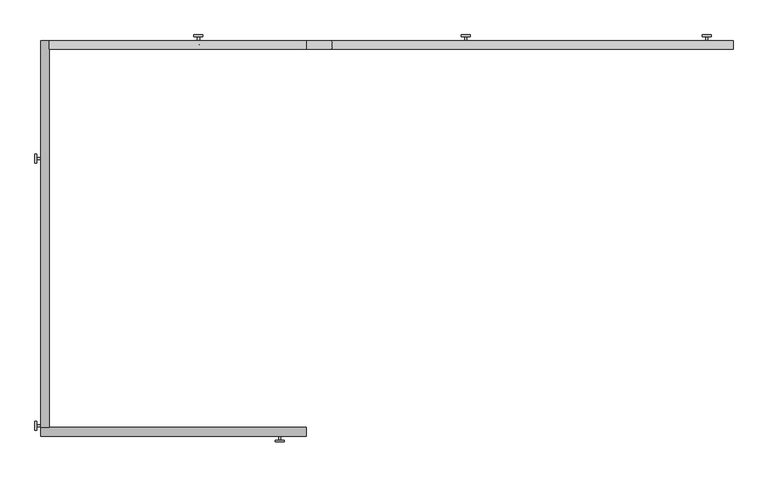
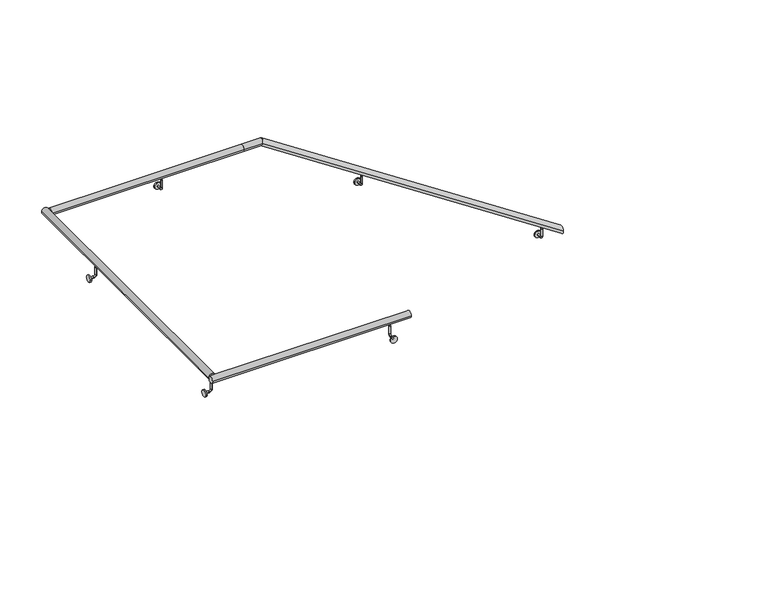
"""IFC4 building model written with IfcOpenShell, lengths in millimetres: railing geometry."""

import ifcopenshell
import ifcopenshell.guid

model = None  # the IFC model being written
_history = None  # IfcOwnerHistory: only IFC2X3 demands one
_inside = {}  # id of a spatial element -> (the spatial element, [elements in it])
_under = {}  # id of a project, library or spatial element -> (it, [spatial elements below it])
_declared = {}  # id of a project -> (the project, [libraries it declares])
_typed = {}  # id of a type object -> (the type object, [elements of that type])
_made_of = {}  # id of a material, layer set ... -> (it, [elements and type objects made of it])


def new_model(schema):
    """Start an empty IFC model of exactly this schema.

    Asked for "IFC4X3", IfcOpenShell would pick the latest addendum, in which some entities
    have other attributes; the version numbers below select the first issue.
    IFC2X3 requires an IfcOwnerHistory on every rooted entity: one is made here for all.
    """
    global model, _history
    if schema == "IFC4X3":
        model = ifcopenshell.file(schema_version=(4, 3, 0, 0))
    else:
        model = ifcopenshell.file(schema=schema)
    _inside.clear()
    _under.clear()
    _declared.clear()
    _typed.clear()
    _made_of.clear()
    _history = None
    if model.schema == "IFC2X3":
        org = make("IfcOrganization", Name="unknown")
        user = make(
            "IfcPersonAndOrganization",
            ThePerson=make("IfcPerson", FamilyName="unknown"),
            TheOrganization=org,
        )
        app = make(
            "IfcApplication",
            ApplicationDeveloper=org,
            Version="unknown",
            ApplicationFullName="unknown",
            ApplicationIdentifier="unknown",
        )
        _history = make(
            "IfcOwnerHistory",
            OwningUser=user,
            OwningApplication=app,
            ChangeAction="ADDED",
            CreationDate=0,
        )
    return model


def make(cls, **values):
    """One entity of the class cls with the attributes given. An attribute that is None is left unset."""
    return model.create_entity(
        cls, **{name: value for name, value in values.items() if value is not None}
    )


def rooted(cls, **values):
    """An entity with a GlobalId (a new one), such as an element, a storey or a relation."""
    return make(cls, GlobalId=ifcopenshell.guid.new(), OwnerHistory=_history, **values)


def si_unit(unit_type, name, prefix=None):
    """IfcSIUnit, for example si_unit("LENGTHUNIT", "METRE", prefix="MILLI")."""
    return make("IfcSIUnit", UnitType=unit_type, Prefix=prefix, Name=name)


def assignment(units):
    """IfcUnitAssignment: the units of a project."""
    return None if units is None else make("IfcUnitAssignment", Units=units)


def point(xyz):
    """IfcCartesianPoint."""
    return None if xyz is None else make("IfcCartesianPoint", Coordinates=xyz)


def direction(xyz):
    """IfcDirection."""
    return None if xyz is None else make("IfcDirection", DirectionRatios=xyz)


def frame(location, z_axis=None, x_axis=None):
    """IfcAxis2Placement3D, a coordinate frame: its origin and axes. An axis left out is left unset."""
    return make(
        "IfcAxis2Placement3D",
        Location=point(location),
        Axis=direction(z_axis),
        RefDirection=direction(x_axis),
    )


def frame_2d(location, x_axis=None):
    """IfcAxis2Placement2D, a coordinate frame in the plane: its origin and x axis."""
    return make(
        "IfcAxis2Placement2D", Location=point(location), RefDirection=direction(x_axis)
    )


def origin():
    """The frame at (0, 0, 0) with its axes left unset."""
    return frame((0.0, 0.0, 0.0))


def place(relative_to, where):
    """IfcLocalPlacement: puts the frame where relative to a parent placement (None: the world)."""
    return make(
        "IfcLocalPlacement", PlacementRelTo=relative_to, RelativePlacement=where
    )


def context(
    kind, dimensions, precision=None, world=None, true_north=None, identifier=None
):
    """IfcGeometricRepresentationContext, for example the 3D "Model" context."""
    return make(
        "IfcGeometricRepresentationContext",
        ContextIdentifier=identifier,
        ContextType=kind,
        CoordinateSpaceDimension=dimensions,
        Precision=precision,
        WorldCoordinateSystem=world,
        TrueNorth=true_north,
    )


def project(units=None, contexts=None):
    """IfcProject with its units and contexts."""
    return rooted(
        "IfcProject",
        Name="project",
        RepresentationContexts=contexts,
        UnitsInContext=assignment(units),
    )


def spatial(cls, under=None, at=None, **own):
    """A site, building, storey or space (cls), placed at a placement, below another one or the project."""
    s = rooted(cls, ObjectPlacement=at, **own)
    if under is not None:
        _under.setdefault(under.id(), (under, []))[1].append(s)
    return s


def circle_curve(where, radius):
    """IfcCircle in the frame where."""
    return make("IfcCircle", Position=where, Radius=radius)


def ellipse_curve(where, semi_axis1, semi_axis2):
    """IfcEllipse in the frame where."""
    return make(
        "IfcEllipse", Position=where, SemiAxis1=semi_axis1, SemiAxis2=semi_axis2
    )


def trimmed(basis, trim1, trim2, sense, master):
    """IfcTrimmedCurve: the piece of a basis curve between two trims."""
    return make(
        "IfcTrimmedCurve",
        BasisCurve=basis,
        Trim1=trim1,
        Trim2=trim2,
        SenseAgreement=sense,
        MasterRepresentation=master,
    )


def segment(curve, same_sense, transition):
    """IfcCompositeCurveSegment."""
    return make(
        "IfcCompositeCurveSegment",
        Transition=transition,
        SameSense=same_sense,
        ParentCurve=curve,
    )


def composite_curve(segments, self_intersect=None):
    """IfcCompositeCurve: segments joined end to end."""
    return make("IfcCompositeCurve", Segments=segments, SelfIntersect=self_intersect)


def outline(outer, holes=None, kind="AREA"):
    """IfcArbitraryClosedProfileDef: a profile drawn as a closed curve; with holes, ...WithVoids."""
    if holes is None:
        return make("IfcArbitraryClosedProfileDef", ProfileType=kind, OuterCurve=outer)
    return make(
        "IfcArbitraryProfileDefWithVoids",
        ProfileType=kind,
        OuterCurve=outer,
        InnerCurves=holes,
    )


def extrude(swept, where, along, depth):
    """IfcExtrudedAreaSolid: the profile swept, set in the frame where, extruded along a direction by depth."""
    return make(
        "IfcExtrudedAreaSolid",
        SweptArea=swept,
        Position=where,
        ExtrudedDirection=direction(along),
        Depth=depth,
    )


def shape(context_of_items, identifier, shape_type, items):
    """IfcShapeRepresentation: the items that make up one representation, for example the "Body"."""
    return make(
        "IfcShapeRepresentation",
        ContextOfItems=context_of_items,
        RepresentationIdentifier=identifier,
        RepresentationType=shape_type,
        Items=items,
    )


def source(mapping_origin, context_of_items, identifier, shape_type, items):
    """IfcRepresentationMap: a shape defined once, which mapped items show again and again."""
    return make(
        "IfcRepresentationMap",
        MappingOrigin=mapping_origin,
        MappedRepresentation=shape(context_of_items, identifier, shape_type, items),
    )


def transform(
    local_origin,
    x_axis=None,
    y_axis=None,
    z_axis=None,
    scale=None,
    scale2=None,
    scale3=None,
    uniform=True,
):
    """IfcCartesianTransformationOperator3D, or its non-uniform kind. x_axis, y_axis, z_axis: its Axis1, 2, 3."""
    if uniform:
        return make(
            "IfcCartesianTransformationOperator3D",
            Axis1=direction(x_axis),
            Axis2=direction(y_axis),
            LocalOrigin=point(local_origin),
            Scale=scale,
            Axis3=direction(z_axis),
        )
    return make(
        "IfcCartesianTransformationOperator3DnonUniform",
        Axis1=direction(x_axis),
        Axis2=direction(y_axis),
        LocalOrigin=point(local_origin),
        Scale=scale,
        Axis3=direction(z_axis),
        Scale2=scale2,
        Scale3=scale3,
    )


def mapped(mapping_source, mapping_target):
    """IfcMappedItem: shows the shape of a source again, moved by a transform."""
    return make(
        "IfcMappedItem", MappingSource=mapping_source, MappingTarget=mapping_target
    )


def made_of(thing, what):
    """Note that an element or type object is made of a material, layer set ...; save() writes the relation."""
    if what is not None:
        _made_of.setdefault(what.id(), (what, []))[1].append(thing)
    return thing


def element(
    cls,
    number,
    at=None,
    inside=None,
    cuts=None,
    type_object=None,
    material=None,
    context=None,
    identifier="Body",
    shape_type=None,
    held_by="IfcProductDefinitionShape",
    body=None,
    shapes=None,
    **own,
):
    """One element of the class cls, such as IfcWall. Its Tag is "e" and its number.

    at: its placement. inside: the storey or other place that contains it. cuts: it is an
    opening in that element (IfcRelVoidsElement). A single representation is given by context,
    identifier, shape_type and body (its items); several are given by shapes. held_by: the class
    of the entity that holds the representations. save() writes the other relations.
    """
    e = rooted(cls, Tag="e%d" % number, ObjectPlacement=at, **own)
    if body is not None:
        shapes = [shape(context, identifier, shape_type, body)]
    if shapes is not None:
        e.Representation = make(held_by, Representations=shapes)
    if inside is not None:
        _inside.setdefault(inside.id(), (inside, []))[1].append(e)
    if cuts is not None:
        rooted(
            "IfcRelVoidsElement", RelatingBuildingElement=cuts, RelatedOpeningElement=e
        )
    if type_object is not None:
        _typed.setdefault(type_object.id(), (type_object, []))[1].append(e)
    return made_of(e, material)


def aggregate(whole, parts):
    """IfcRelAggregates: a whole, such as a stair, and the parts it consists of."""
    return rooted("IfcRelAggregates", RelatingObject=whole, RelatedObjects=parts)


def save(model, path):
    """Write the relations noted so far, then the file.

    IfcRelAggregates (storeys below a building ...), IfcRelContainedInSpatialStructure (elements
    in a storey), IfcRelDefinesByType, IfcRelAssociatesMaterial and IfcRelDeclares: one each for
    every whole, place, type object, material and project.
    """
    for whole, parts in _under.values():
        aggregate(whole, parts)
    for where, things in _inside.values():
        rooted(
            "IfcRelContainedInSpatialStructure",
            RelatedElements=things,
            RelatingStructure=where,
        )
    for kind, things in _typed.values():
        rooted("IfcRelDefinesByType", RelatedObjects=things, RelatingType=kind)
    for what, things in _made_of.values():
        rooted("IfcRelAssociatesMaterial", RelatedObjects=things, RelatingMaterial=what)
    for by, libraries in _declared.values():
        rooted("IfcRelDeclares", RelatingContext=by, RelatedDefinitions=libraries)
    model.write(path)


def plane_surface(at):
    """IfcPlane: the flat surface through the origin of the frame at, square to its z axis."""
    return make("IfcPlane", Position=at)


def cylinder_surface(at, radius):
    """IfcCylindricalSurface: all points at the distance radius from the z axis of the frame at."""
    return make("IfcCylindricalSurface", Position=at, Radius=radius)


def revolved_surface(curve, axis_point, axis_direction):
    """IfcSurfaceOfRevolution: the curve turned about the line through axis_point along axis_direction."""
    return make(
        "IfcSurfaceOfRevolution",
        SweptCurve=make("IfcArbitraryOpenProfileDef", ProfileType="CURVE", Curve=curve),
        AxisPosition=make("IfcAxis1Placement", Location=point(axis_point), Axis=direction(axis_direction)),
    )


def advanced_brep(points, edges, surfaces, faces):
    """IfcAdvancedBrep: a solid bounded by faces that lie on surfaces and meet in shared edges.

    An edge is (start, end): straight between two places in points (the first is 0);
    or (start, end, curve); or (start, end, curve, False) where it runs against its curve.
    A face is (place in surfaces, loops), or (place, loops, False) where it looks against
    its surface's normal. A loop lists edges by number (the first is 1), with a minus sign
    where the edge is run from its end to its start. The first loop is the outer one.
    """
    corners = [point(p) for p in points]
    vertices = [make("IfcVertexPoint", VertexGeometry=c) for c in corners]
    made = []
    for start, end, *more in edges:
        made.append(
            make(
                "IfcEdgeCurve",
                EdgeStart=vertices[start],
                EdgeEnd=vertices[end],
                EdgeGeometry=more[0] if more else make("IfcPolyline", Points=[corners[start], corners[end]]),
                SameSense=more[1] if len(more) > 1 else True,
            )
        )
    hull = []
    for where, loops, *sense in faces:
        bounds = []
        for j, loop in enumerate(loops):
            ring = [make("IfcOrientedEdge", EdgeElement=made[abs(k) - 1], Orientation=k > 0) for k in loop]
            bounds.append(
                make(
                    "IfcFaceOuterBound" if j == 0 else "IfcFaceBound",
                    Bound=make("IfcEdgeLoop", EdgeList=ring),
                    Orientation=True,
                )
            )
        hull.append(make("IfcAdvancedFace", Bounds=bounds, FaceSurface=surfaces[where], SameSense=sense[0] if sense else True))
    return make("IfcAdvancedBrep", Outer=make("IfcClosedShell", CfsFaces=hull))


def railing_9a7f1ff8(model_context):
    return source(origin(), model_context, "Body", "SolidModel", [
        advanced_brep(
        [(-47571.8499394, -5172.6994487, 1246.5391039), (-47571.8499394, -5122.6994487, 1246.5391039), (-49859.4499252, -5172.6994487, 2752.7777778), (-49859.4499252, -5122.6994487, 2752.7777778), (-50001.8499394, -5172.6994487, 2752.7777778), (-50001.8499394, -5122.6994487, 2752.7777778)],
        [
            (0, 1, ellipse_curve(frame((-47571.8499394, -5147.6994487, 1246.5391039), z_axis=(1.0, 0.0, 0.0), x_axis=(0.0, 0.0, -1.0)), 29.9326144, 25.0)),
            (1, 0, ellipse_curve(frame((-47571.8499394, -5147.6994487, 1246.5391039), z_axis=(1.0, 0.0, 0.0), x_axis=(0.0, 0.0, -1.0)), 29.9326144, 25.0)),
            (0, 2),
            (2, 3, ellipse_curve(frame((-49859.4499252, -5147.6994487, 2752.7777778), z_axis=(0.9579168464509247, 0.0, -0.28704584178405307), x_axis=(-0.2870458417840529, 0.0, -0.9579168464509247)), 26.0982987, 25.0)),
            (3, 1),
            (3, 2, ellipse_curve(frame((-49859.4499252, -5147.6994487, 2752.7777778), z_axis=(0.9579168464509247, 0.0, -0.28704584178405307), x_axis=(-0.2870458417840529, 0.0, -0.9579168464509247)), 26.0982987, 25.0)),
            (4, 5, circle_curve(frame((-50001.8499394, -5147.6994487, 2752.7777778), z_axis=(-1.0, 0.0, 0.0), x_axis=(0.0, 1.0, 0.0)), 25.0)),
            (5, 4, circle_curve(frame((-50001.8499394, -5147.6994487, 2752.7777778), z_axis=(-1.0, 0.0, 0.0), x_axis=(0.0, 1.0, 0.0)), 25.0)),
            (2, 4),
            (5, 3),
        ],
        [
            plane_surface(frame((-47571.8499394, -5147.6994487, 1276.4717183), z_axis=(1.0, 0.0, 0.0), x_axis=(0.0, -1.0, 0.0))),
            cylinder_surface(frame((-47585.5982417, -5147.6994487, 1255.5914841), z_axis=(0.8352093694289688, 0.0, -0.5499320950972624), x_axis=(0.0, 1.0, 0.0)), 25.0),
            plane_surface(frame((-50001.8499394, -5147.6994487, 2777.7777778), z_axis=(-1.0, 0.0, 0.0), x_axis=(0.0, -1.0, 0.0))),
            cylinder_surface(frame((-49851.9585171, -5147.6994487, 2752.7777778), z_axis=(1.0, 0.0, 0.0), x_axis=(0.0, 1.0, 0.0)), 25.0),
        ],
        [
            (0, [[1, 2]]),
            (1, [[-1, 3, 4, 5]]),
            (1, [[-2, -5, 6, -3]]),
            (2, [[7, 8]]),
            (3, [[-4, 9, -8, 10]]),
            (3, [[-6, -10, -7, -9]]),
        ],
    ),
        advanced_brep(
        [(-50001.8499394, -5172.6994487, 2752.7777778), (-50001.8499394, -5122.6994487, 2752.7777778), (-51463.5128792, -5172.6994487, 2752.7777778), (-51463.5128792, -5122.6994487, 2752.7777778)],
        [
            (0, 1, circle_curve(frame((-50001.8499394, -5147.6994487, 2752.7777778), z_axis=(1.0, 0.0, 0.0), x_axis=(0.0, 1.0, 0.0)), 25.0)),
            (1, 0, circle_curve(frame((-50001.8499394, -5147.6994487, 2752.7777778), z_axis=(1.0, 0.0, 0.0), x_axis=(0.0, 1.0, 0.0)), 25.0)),
            (2, 3, circle_curve(frame((-51463.5128792, -5147.6994487, 2752.7777778), z_axis=(-1.0, 0.0, 0.0), x_axis=(0.0, 1.0, 0.0)), 25.0)),
            (3, 2, circle_curve(frame((-51463.5128792, -5147.6994487, 2752.7777778), z_axis=(-1.0, 0.0, 0.0), x_axis=(0.0, 1.0, 0.0)), 25.0)),
            (0, 2),
            (3, 1),
        ],
        [
            plane_surface(frame((-50001.8499394, -5147.6994487, 2777.7777778), z_axis=(1.0, 0.0, 0.0), x_axis=(0.0, -1.0, 0.0))),
            plane_surface(frame((-51463.5128792, -5147.6994487, 2777.7777778), z_axis=(-1.0, 0.0, 0.0), x_axis=(0.0, -1.0, 0.0))),
            cylinder_surface(frame((-50001.8499394, -5147.6994487, 2752.7777778), z_axis=(1.0, 0.0, 0.0), x_axis=(0.0, 1.0, 0.0)), 25.0),
        ],
        [
            (0, [[1, 2]]),
            (1, [[3, 4]]),
            (2, [[-1, 5, -4, 6]]),
            (2, [[-2, -6, -3, -5]]),
        ],
    ),
        advanced_brep(
        [(-51463.5128792, -5122.6994487, 2752.7777778), (-51513.5128792, -5122.6994487, 2752.7777778), (-51463.5128792, -7327.4994487, 2752.7777778), (-51513.5128792, -7327.4994487, 2752.7777778)],
        [
            (0, 1, circle_curve(frame((-51488.5128792, -5122.6994487, 2752.7777778), z_axis=(0.0, 1.0, 0.0), x_axis=(-1.0, 0.0, 0.0)), 25.0)),
            (1, 0, circle_curve(frame((-51488.5128792, -5122.6994487, 2752.7777778), z_axis=(0.0, 1.0, 0.0), x_axis=(-1.0, 0.0, 0.0)), 25.0)),
            (2, 3, circle_curve(frame((-51488.5128792, -7327.4994487, 2752.7777778), z_axis=(0.0, -1.0, 0.0), x_axis=(-1.0, 0.0, 0.0)), 25.0)),
            (3, 2, circle_curve(frame((-51488.5128792, -7327.4994487, 2752.7777778), z_axis=(0.0, -1.0, 0.0), x_axis=(-1.0, 0.0, 0.0)), 25.0)),
            (0, 2),
            (3, 1),
        ],
        [
            plane_surface(frame((-51488.5128792, -5122.6994487, 2777.7777778), z_axis=(0.0, 1.0, 0.0), x_axis=(0.0, 0.0, -1.0))),
            plane_surface(frame((-51488.5128792, -7327.4994487, 2777.7777778), z_axis=(0.0, -1.0, 0.0), x_axis=(0.0, 0.0, -1.0))),
            cylinder_surface(frame((-51488.5128792, -5122.6994487, 2752.7777778), z_axis=(0.0, 1.0, 0.0), x_axis=(-1.0, 0.0, 0.0)), 25.0),
        ],
        [
            (0, [[1, 2]]),
            (1, [[3, 4]]),
            (2, [[-1, 5, -4, 6]]),
            (2, [[-2, -6, -3, -5]]),
        ],
    ),
        advanced_brep(
        [(-51513.5128792, -7327.4994487, 2752.7777778), (-51513.5128792, -7377.4994487, 2752.7777778), (-50001.8499394, -7327.4994487, 2752.7777778), (-50001.8499394, -7377.4994487, 2752.7777778)],
        [
            (0, 1, circle_curve(frame((-51513.5128792, -7352.4994487, 2752.7777778), z_axis=(-1.0, 0.0, 0.0), x_axis=(0.0, -1.0, 0.0)), 25.0)),
            (1, 0, circle_curve(frame((-51513.5128792, -7352.4994487, 2752.7777778), z_axis=(-1.0, 0.0, 0.0), x_axis=(0.0, -1.0, 0.0)), 25.0)),
            (2, 3, circle_curve(frame((-50001.8499394, -7352.4994487, 2752.7777778), z_axis=(1.0, 0.0, 0.0), x_axis=(0.0, -1.0, 0.0)), 25.0)),
            (3, 2, circle_curve(frame((-50001.8499394, -7352.4994487, 2752.7777778), z_axis=(1.0, 0.0, 0.0), x_axis=(0.0, -1.0, 0.0)), 25.0)),
            (0, 2),
            (3, 1),
        ],
        [
            plane_surface(frame((-51513.5128792, -7352.4994487, 2777.7777778), z_axis=(-1.0, 0.0, 0.0), x_axis=(0.0, 1.0, 0.0))),
            plane_surface(frame((-50001.8499394, -7352.4994487, 2777.7777778), z_axis=(1.0, 0.0, 0.0), x_axis=(0.0, 1.0, 0.0))),
            cylinder_surface(frame((-51513.5128792, -7352.4994487, 2752.7777778), z_axis=(-1.0, 0.0, 0.0), x_axis=(0.0, -1.0, 0.0)), 25.0),
        ],
        [
            (0, [[1, 2]]),
            (1, [[3, 4]]),
            (2, [[-1, 5, -4, 6]]),
            (2, [[-2, -6, -3, -5]]),
        ],
    ),
        advanced_brep(
        [(-51488.5128792, -7311.1872126, 2708.7277778), (-51488.5128792, -7323.8872126, 2708.7277778), (-51488.5128792, -7311.1872126, 2651.5777778), (-51488.5128792, -7323.8872126, 2651.5777778), (-51507.5628792, -7323.8872126, 2632.5277778), (-51507.5628792, -7311.1872126, 2632.5277778), (-51536.1378792, -7311.1872126, 2632.5277778), (-51536.1378792, -7323.8872126, 2632.5277778)],
        [
            (0, 1, circle_curve(frame((-51488.5128792, -7317.5372126, 2708.7277778), z_axis=(0.0, 0.0, 1.0), x_axis=(0.0, -1.0, 0.0)), 6.35)),
            (1, 0, circle_curve(frame((-51488.5128792, -7317.5372126, 2708.7277778), z_axis=(0.0, 0.0, 1.0), x_axis=(0.0, -1.0, 0.0)), 6.35)),
            (0, 2),
            (2, 3, circle_curve(frame((-51488.5128792, -7317.5372126, 2651.5777778), z_axis=(0.0, 0.0, 1.0), x_axis=(0.0, -1.0, 0.0)), 6.35)),
            (3, 1),
            (3, 2, circle_curve(frame((-51488.5128792, -7317.5372126, 2651.5777778), z_axis=(0.0, 0.0, 1.0), x_axis=(0.0, -1.0, 0.0)), 6.35)),
            (4, 3, circle_curve(frame((-51507.5628792, -7323.8872126, 2651.5777778), z_axis=(0.0, -1.0, 0.0), x_axis=(1.0, 0.0, 0.0)), 19.05)),
            (2, 5, circle_curve(frame((-51507.5628792, -7311.1872126, 2651.5777778), z_axis=(0.0, 1.0, 0.0), x_axis=(1.0, 0.0, 0.0)), 19.05)),
            (5, 4, circle_curve(frame((-51507.5628792, -7317.5372126, 2632.5277778), z_axis=(1.0, 0.0, 0.0), x_axis=(0.0, -1.0, 0.0)), 6.35)),
            (4, 5, circle_curve(frame((-51507.5628792, -7317.5372126, 2632.5277778), z_axis=(1.0, 0.0, 0.0), x_axis=(0.0, -1.0, 0.0)), 6.35)),
            (6, 7, circle_curve(frame((-51536.1378792, -7317.5372126, 2632.5277778), z_axis=(-1.0, 0.0, 0.0), x_axis=(0.0, -1.0, 0.0)), 6.35)),
            (7, 6, circle_curve(frame((-51536.1378792, -7317.5372126, 2632.5277778), z_axis=(-1.0, 0.0, 0.0), x_axis=(0.0, -1.0, 0.0)), 6.35)),
            (5, 6),
            (7, 4),
        ],
        [
            plane_surface(frame((-51488.5128792, -7323.8872126, 2708.7277778), z_axis=(0.0, 0.0, 1.0), x_axis=(-1.0, 0.0, 0.0))),
            cylinder_surface(frame((-51488.5128792, -7317.5372126, 2708.7277778), z_axis=(0.0, 0.0, 1.0), x_axis=(0.0, -1.0, 0.0)), 6.35),
            revolved_surface(trimmed(ellipse_curve(frame((-51488.5128792, -7317.5372126, 2651.5777778), z_axis=(0.0, 0.0, 1.0), x_axis=(0.0, -1.0, 0.0)), 6.35, 6.35), [point((-51488.5128792, -7311.1872126, 2651.5777778))], [point((-51488.5128792, -7323.8872126, 2651.5777778))], True, "CARTESIAN"), (-51507.5628792, -7317.5372126, 2651.5777778), (0.0, 1.0, 0.0)),
            revolved_surface(trimmed(ellipse_curve(frame((-51488.5128792, -7317.5372126, 2651.5777778), z_axis=(0.0, 0.0, 1.0), x_axis=(0.0, -1.0, 0.0)), 6.35, 6.35), [point((-51488.5128792, -7323.8872126, 2651.5777778))], [point((-51488.5128792, -7311.1872126, 2651.5777778))], True, "CARTESIAN"), (-51507.5628792, -7317.5372126, 2651.5777778), (0.0, 1.0, 0.0)),
            plane_surface(frame((-51536.1378792, -7317.5372126, 2626.1777778), z_axis=(-1.0, 0.0, 0.0), x_axis=(0.0, -1.0, 0.0))),
            cylinder_surface(frame((-51507.5628792, -7317.5372126, 2632.5277778), z_axis=(1.0, 0.0, 0.0), x_axis=(0.0, -1.0, 0.0)), 6.35),
        ],
        [
            (0, [[1, 2]]),
            (1, [[-1, 3, 4, 5]]),
            (1, [[-2, -5, 6, -3]]),
            (2, [[7, -4, 8, 9]]),
            (3, [[-8, -6, -7, 10]]),
            (4, [[11, 12]]),
            (5, [[-9, 13, -12, 14]]),
            (5, [[-10, -14, -11, -13]]),
        ],
    ),
        extrude(outline(composite_curve([segment(trimmed(circle_curve(frame_2d((-7317.5372126, 2632.5277778)), 25.4), [point((-7342.9372126, 2632.5277778))], [point((-7292.1372126, 2632.5277778))], False, "CARTESIAN"), True, "CONTINUOUS"), segment(trimmed(circle_curve(frame_2d((-7317.5372126, 2632.5277778)), 25.4), [point((-7292.1372126, 2632.5277778))], [point((-7342.9372126, 2632.5277778))], False, "CARTESIAN"), True, "CONTINUOUS")], self_intersect=False)), frame((-51545.6628792, 0.0, 0.0), z_axis=(1.0, 0.0, 0.0), x_axis=(0.0, 1.0, 0.0)), (0.0, 0.0, 1.0), 9.525),
        advanced_brep(
        [(-51488.5128792, -5789.5620366, 2708.7277778), (-51488.5128792, -5802.2620366, 2708.7277778), (-51488.5128792, -5789.5620366, 2651.5777778), (-51488.5128792, -5802.2620366, 2651.5777778), (-51507.5628792, -5802.2620366, 2632.5277778), (-51507.5628792, -5789.5620366, 2632.5277778), (-51536.1378792, -5789.5620366, 2632.5277778), (-51536.1378792, -5802.2620366, 2632.5277778)],
        [
            (0, 1, circle_curve(frame((-51488.5128792, -5795.9120366, 2708.7277778), z_axis=(0.0, 0.0, 1.0), x_axis=(0.0, -1.0, 0.0)), 6.35)),
            (1, 0, circle_curve(frame((-51488.5128792, -5795.9120366, 2708.7277778), z_axis=(0.0, 0.0, 1.0), x_axis=(0.0, -1.0, 0.0)), 6.35)),
            (0, 2),
            (2, 3, circle_curve(frame((-51488.5128792, -5795.9120366, 2651.5777778), z_axis=(0.0, 0.0, 1.0), x_axis=(0.0, -1.0, 0.0)), 6.35)),
            (3, 1),
            (3, 2, circle_curve(frame((-51488.5128792, -5795.9120366, 2651.5777778), z_axis=(0.0, 0.0, 1.0), x_axis=(0.0, -1.0, 0.0)), 6.35)),
            (4, 3, circle_curve(frame((-51507.5628792, -5802.2620366, 2651.5777778), z_axis=(0.0, -1.0, 0.0), x_axis=(1.0, 0.0, 0.0)), 19.05)),
            (2, 5, circle_curve(frame((-51507.5628792, -5789.5620366, 2651.5777778), z_axis=(0.0, 1.0, 0.0), x_axis=(1.0, 0.0, 0.0)), 19.05)),
            (5, 4, circle_curve(frame((-51507.5628792, -5795.9120366, 2632.5277778), z_axis=(1.0, 0.0, 0.0), x_axis=(0.0, -1.0, 0.0)), 6.35)),
            (4, 5, circle_curve(frame((-51507.5628792, -5795.9120366, 2632.5277778), z_axis=(1.0, 0.0, 0.0), x_axis=(0.0, -1.0, 0.0)), 6.35)),
            (6, 7, circle_curve(frame((-51536.1378792, -5795.9120366, 2632.5277778), z_axis=(-1.0, 0.0, 0.0), x_axis=(0.0, -1.0, 0.0)), 6.35)),
            (7, 6, circle_curve(frame((-51536.1378792, -5795.9120366, 2632.5277778), z_axis=(-1.0, 0.0, 0.0), x_axis=(0.0, -1.0, 0.0)), 6.35)),
            (5, 6),
            (7, 4),
        ],
        [
            plane_surface(frame((-51488.5128792, -5802.2620366, 2708.7277778), z_axis=(0.0, 0.0, 1.0), x_axis=(-1.0, 0.0, 0.0))),
            cylinder_surface(frame((-51488.5128792, -5795.9120366, 2708.7277778), z_axis=(0.0, 0.0, 1.0), x_axis=(0.0, -1.0, 0.0)), 6.35),
            revolved_surface(trimmed(ellipse_curve(frame((-51488.5128792, -5795.9120366, 2651.5777778), z_axis=(0.0, 0.0, 1.0), x_axis=(0.0, -1.0, 0.0)), 6.35, 6.35), [point((-51488.5128792, -5789.5620366, 2651.5777778))], [point((-51488.5128792, -5802.2620366, 2651.5777778))], True, "CARTESIAN"), (-51507.5628792, -5795.9120366, 2651.5777778), (0.0, 1.0, 0.0)),
            revolved_surface(trimmed(ellipse_curve(frame((-51488.5128792, -5795.9120366, 2651.5777778), z_axis=(0.0, 0.0, 1.0), x_axis=(0.0, -1.0, 0.0)), 6.35, 6.35), [point((-51488.5128792, -5802.2620366, 2651.5777778))], [point((-51488.5128792, -5789.5620366, 2651.5777778))], True, "CARTESIAN"), (-51507.5628792, -5795.9120366, 2651.5777778), (0.0, 1.0, 0.0)),
            plane_surface(frame((-51536.1378792, -5795.9120366, 2626.1777778), z_axis=(-1.0, 0.0, 0.0), x_axis=(0.0, -1.0, 0.0))),
            cylinder_surface(frame((-51507.5628792, -5795.9120366, 2632.5277778), z_axis=(1.0, 0.0, 0.0), x_axis=(0.0, -1.0, 0.0)), 6.35),
        ],
        [
            (0, [[1, 2]]),
            (1, [[-1, 3, 4, 5]]),
            (1, [[-2, -5, 6, -3]]),
            (2, [[7, -4, 8, 9]]),
            (3, [[-8, -6, -7, 10]]),
            (4, [[11, 12]]),
            (5, [[-9, 13, -12, 14]]),
            (5, [[-10, -14, -11, -13]]),
        ],
    ),
        extrude(outline(composite_curve([segment(trimmed(circle_curve(frame_2d((-5795.9120366, 2632.5277778)), 25.4), [point((-5821.3120366, 2632.5277778))], [point((-5770.5120366, 2632.5277778))], False, "CARTESIAN"), True, "CONTINUOUS"), segment(trimmed(circle_curve(frame_2d((-5795.9120366, 2632.5277778)), 25.4), [point((-5770.5120366, 2632.5277778))], [point((-5821.3120366, 2632.5277778))], False, "CARTESIAN"), True, "CONTINUOUS")], self_intersect=False)), frame((-51545.6628792, 0.0, 0.0), z_axis=(1.0, 0.0, 0.0), x_axis=(0.0, 1.0, 0.0)), (0.0, 0.0, 1.0), 9.525),
        advanced_brep(
        [(-50608.7502912, -5147.6994487, 2708.7277778), (-50621.4502912, -5147.6994487, 2708.7277778), (-50608.7502912, -5147.6994487, 2651.5777778), (-50621.4502912, -5147.6994487, 2651.5777778), (-50621.4502912, -5128.6494487, 2632.5277778), (-50608.7502912, -5128.6494487, 2632.5277778), (-50608.7502912, -5100.0744487, 2632.5277778), (-50621.4502912, -5100.0744487, 2632.5277778)],
        [
            (0, 1, circle_curve(frame((-50615.1002912, -5147.6994487, 2708.7277778), z_axis=(0.0, 0.0, 1.0), x_axis=(-1.0, 0.0, 0.0)), 6.35)),
            (1, 0, circle_curve(frame((-50615.1002912, -5147.6994487, 2708.7277778), z_axis=(0.0, 0.0, 1.0), x_axis=(-1.0, 0.0, 0.0)), 6.35)),
            (0, 2),
            (2, 3, circle_curve(frame((-50615.1002912, -5147.6994487, 2651.5777778), z_axis=(0.0, 0.0, 1.0), x_axis=(-1.0, 0.0, 0.0)), 6.35)),
            (3, 1),
            (3, 2, circle_curve(frame((-50615.1002912, -5147.6994487, 2651.5777778), z_axis=(0.0, 0.0, 1.0), x_axis=(-1.0, 0.0, 0.0)), 6.35)),
            (4, 3, circle_curve(frame((-50621.4502912, -5128.6494487, 2651.5777778), z_axis=(-1.0, 0.0, 0.0), x_axis=(0.0, -1.0, 0.0)), 19.05)),
            (2, 5, circle_curve(frame((-50608.7502912, -5128.6494487, 2651.5777778), z_axis=(1.0, 0.0, 0.0), x_axis=(0.0, -1.0, 0.0)), 19.05)),
            (5, 4, circle_curve(frame((-50615.1002912, -5128.6494487, 2632.5277778), z_axis=(0.0, -1.0, 0.0), x_axis=(-1.0, 0.0, 0.0)), 6.35)),
            (4, 5, circle_curve(frame((-50615.1002912, -5128.6494487, 2632.5277778), z_axis=(0.0, -1.0, 0.0), x_axis=(-1.0, 0.0, 0.0)), 6.35)),
            (6, 7, circle_curve(frame((-50615.1002912, -5100.0744487, 2632.5277778), z_axis=(0.0, 1.0, 0.0), x_axis=(-1.0, 0.0, 0.0)), 6.35)),
            (7, 6, circle_curve(frame((-50615.1002912, -5100.0744487, 2632.5277778), z_axis=(0.0, 1.0, 0.0), x_axis=(-1.0, 0.0, 0.0)), 6.35)),
            (5, 6),
            (7, 4),
        ],
        [
            plane_surface(frame((-50621.4502912, -5147.6994487, 2708.7277778), z_axis=(0.0, 0.0, 1.0), x_axis=(0.0, 1.0, 0.0))),
            cylinder_surface(frame((-50615.1002912, -5147.6994487, 2708.7277778), z_axis=(0.0, 0.0, 1.0), x_axis=(-1.0, 0.0, 0.0)), 6.35),
            revolved_surface(trimmed(ellipse_curve(frame((-50615.1002912, -5147.6994487, 2651.5777778), z_axis=(0.0, 0.0, 1.0), x_axis=(-1.0, 0.0, 0.0)), 6.35, 6.35), [point((-50608.7502912, -5147.6994487, 2651.5777778))], [point((-50621.4502912, -5147.6994487, 2651.5777778))], True, "CARTESIAN"), (-50615.1002912, -5128.6494487, 2651.5777778), (1.0, 0.0, 0.0)),
            revolved_surface(trimmed(ellipse_curve(frame((-50615.1002912, -5147.6994487, 2651.5777778), z_axis=(0.0, 0.0, 1.0), x_axis=(-1.0, 0.0, 0.0)), 6.35, 6.35), [point((-50621.4502912, -5147.6994487, 2651.5777778))], [point((-50608.7502912, -5147.6994487, 2651.5777778))], True, "CARTESIAN"), (-50615.1002912, -5128.6494487, 2651.5777778), (1.0, 0.0, 0.0)),
            plane_surface(frame((-50615.1002912, -5100.0744487, 2626.1777778), z_axis=(0.0, 1.0, 0.0), x_axis=(-1.0, 0.0, 0.0))),
            cylinder_surface(frame((-50615.1002912, -5128.6494487, 2632.5277778), z_axis=(0.0, -1.0, 0.0), x_axis=(-1.0, 0.0, 0.0)), 6.35),
        ],
        [
            (0, [[1, 2]]),
            (1, [[-1, 3, 4, 5]]),
            (1, [[-2, -5, 6, -3]]),
            (2, [[7, -4, 8, 9]]),
            (3, [[-8, -6, -7, 10]]),
            (4, [[11, 12]]),
            (5, [[-9, 13, -12, 14]]),
            (5, [[-10, -14, -11, -13]]),
        ],
    ),
        extrude(outline(composite_curve([segment(trimmed(circle_curve(frame_2d((2632.5277778, -50615.1002912)), 25.4), [point((2632.5277778, -50640.5002912))], [point((2632.5277778, -50589.7002912))], False, "CARTESIAN"), True, "CONTINUOUS"), segment(trimmed(circle_curve(frame_2d((2632.5277778, -50615.1002912)), 25.4), [point((2632.5277778, -50589.7002912))], [point((2632.5277778, -50640.5002912))], False, "CARTESIAN"), True, "CONTINUOUS")], self_intersect=False)), frame((0.0, -5100.0744487, 0.0), z_axis=(0.0, 1.0, 0.0), x_axis=(0.0, 0.0, 1.0)), (0.0, 0.0, 1.0), 9.525),
        advanced_brep(
        [(-49087.1251153, -5147.6994487, 2209.3148383), (-49099.8251153, -5147.6994487, 2209.3148383), (-49087.1251153, -5147.6994487, 2152.1648383), (-49099.8251153, -5147.6994487, 2152.1648383), (-49099.8251153, -5128.6494487, 2133.1148383), (-49087.1251153, -5128.6494487, 2133.1148383), (-49087.1251153, -5100.0744487, 2133.1148383), (-49099.8251153, -5100.0744487, 2133.1148383)],
        [
            (0, 1, circle_curve(frame((-49093.4751153, -5147.6994487, 2209.3148383), z_axis=(0.0, 0.0, 1.0), x_axis=(-1.0, 0.0, 0.0)), 6.35)),
            (1, 0, circle_curve(frame((-49093.4751153, -5147.6994487, 2209.3148383), z_axis=(0.0, 0.0, 1.0), x_axis=(-1.0, 0.0, 0.0)), 6.35)),
            (0, 2),
            (2, 3, circle_curve(frame((-49093.4751153, -5147.6994487, 2152.1648383), z_axis=(0.0, 0.0, 1.0), x_axis=(-1.0, 0.0, 0.0)), 6.35)),
            (3, 1),
            (3, 2, circle_curve(frame((-49093.4751153, -5147.6994487, 2152.1648383), z_axis=(0.0, 0.0, 1.0), x_axis=(-1.0, 0.0, 0.0)), 6.35)),
            (4, 3, circle_curve(frame((-49099.8251153, -5128.6494487, 2152.1648383), z_axis=(-1.0, 0.0, 0.0), x_axis=(0.0, -1.0, 0.0)), 19.05)),
            (2, 5, circle_curve(frame((-49087.1251153, -5128.6494487, 2152.1648383), z_axis=(1.0, 0.0, 0.0), x_axis=(0.0, -1.0, 0.0)), 19.05)),
            (5, 4, circle_curve(frame((-49093.4751153, -5128.6494487, 2133.1148383), z_axis=(0.0, -1.0, 0.0), x_axis=(-1.0, 0.0, 0.0)), 6.35)),
            (4, 5, circle_curve(frame((-49093.4751153, -5128.6494487, 2133.1148383), z_axis=(0.0, -1.0, 0.0), x_axis=(-1.0, 0.0, 0.0)), 6.35)),
            (6, 7, circle_curve(frame((-49093.4751153, -5100.0744487, 2133.1148383), z_axis=(0.0, 1.0, 0.0), x_axis=(-1.0, 0.0, 0.0)), 6.35)),
            (7, 6, circle_curve(frame((-49093.4751153, -5100.0744487, 2133.1148383), z_axis=(0.0, 1.0, 0.0), x_axis=(-1.0, 0.0, 0.0)), 6.35)),
            (5, 6),
            (7, 4),
        ],
        [
            plane_surface(frame((-49099.8251153, -5147.6994487, 2209.3148383), z_axis=(0.0, 0.0, 1.0), x_axis=(0.0, 1.0, 0.0))),
            cylinder_surface(frame((-49093.4751153, -5147.6994487, 2209.3148383), z_axis=(0.0, 0.0, 1.0), x_axis=(-1.0, 0.0, 0.0)), 6.35),
            revolved_surface(trimmed(ellipse_curve(frame((-49093.4751153, -5147.6994487, 2152.1648383), z_axis=(0.0, 0.0, 1.0), x_axis=(-1.0, 0.0, 0.0)), 6.35, 6.35), [point((-49087.1251153, -5147.6994487, 2152.1648383))], [point((-49099.8251153, -5147.6994487, 2152.1648383))], True, "CARTESIAN"), (-49093.4751153, -5128.6494487, 2152.1648383), (1.0, 0.0, 0.0)),
            revolved_surface(trimmed(ellipse_curve(frame((-49093.4751153, -5147.6994487, 2152.1648383), z_axis=(0.0, 0.0, 1.0), x_axis=(-1.0, 0.0, 0.0)), 6.35, 6.35), [point((-49099.8251153, -5147.6994487, 2152.1648383))], [point((-49087.1251153, -5147.6994487, 2152.1648383))], True, "CARTESIAN"), (-49093.4751153, -5128.6494487, 2152.1648383), (1.0, 0.0, 0.0)),
            plane_surface(frame((-49093.4751153, -5100.0744487, 2126.7648383), z_axis=(0.0, 1.0, 0.0), x_axis=(-1.0, 0.0, 0.0))),
            cylinder_surface(frame((-49093.4751153, -5128.6494487, 2133.1148383), z_axis=(0.0, -1.0, 0.0), x_axis=(-1.0, 0.0, 0.0)), 6.35),
        ],
        [
            (0, [[1, 2]]),
            (1, [[-1, 3, 4, 5]]),
            (1, [[-2, -5, 6, -3]]),
            (2, [[7, -4, 8, 9]]),
            (3, [[-8, -6, -7, 10]]),
            (4, [[11, 12]]),
            (5, [[-9, 13, -12, 14]]),
            (5, [[-10, -14, -11, -13]]),
        ],
    ),
        extrude(outline(composite_curve([segment(trimmed(circle_curve(frame_2d((2133.1148383, -49093.4751153)), 25.4), [point((2133.1148383, -49118.8751153))], [point((2133.1148383, -49068.0751153))], False, "CARTESIAN"), True, "CONTINUOUS"), segment(trimmed(circle_curve(frame_2d((2133.1148383, -49093.4751153)), 25.4), [point((2133.1148383, -49068.0751153))], [point((2133.1148383, -49118.8751153))], False, "CARTESIAN"), True, "CONTINUOUS")], self_intersect=False)), frame((0.0, -5100.0744487, 0.0), z_axis=(0.0, 1.0, 0.0), x_axis=(0.0, 0.0, 1.0)), (0.0, 0.0, 1.0), 9.525),
        advanced_brep(
        [(-50158.1999394, -7352.4994487, 2708.7277778), (-50145.4999394, -7352.4994487, 2708.7277778), (-50158.1999394, -7352.4994487, 2651.5777778), (-50145.4999394, -7352.4994487, 2651.5777778), (-50145.4999394, -7371.5494487, 2632.5277778), (-50158.1999394, -7371.5494487, 2632.5277778), (-50158.1999394, -7400.1244487, 2632.5277778), (-50145.4999394, -7400.1244487, 2632.5277778)],
        [
            (0, 1, circle_curve(frame((-50151.8499394, -7352.4994487, 2708.7277778), z_axis=(0.0, 0.0, 1.0), x_axis=(1.0, 0.0, 0.0)), 6.35)),
            (1, 0, circle_curve(frame((-50151.8499394, -7352.4994487, 2708.7277778), z_axis=(0.0, 0.0, 1.0), x_axis=(1.0, 0.0, 0.0)), 6.35)),
            (0, 2),
            (2, 3, circle_curve(frame((-50151.8499394, -7352.4994487, 2651.5777778), z_axis=(0.0, 0.0, 1.0), x_axis=(1.0, 0.0, 0.0)), 6.35)),
            (3, 1),
            (3, 2, circle_curve(frame((-50151.8499394, -7352.4994487, 2651.5777778), z_axis=(0.0, 0.0, 1.0), x_axis=(1.0, 0.0, 0.0)), 6.35)),
            (4, 3, circle_curve(frame((-50145.4999394, -7371.5494487, 2651.5777778), z_axis=(1.0, 0.0, 0.0), x_axis=(0.0, 1.0, 0.0)), 19.05)),
            (2, 5, circle_curve(frame((-50158.1999394, -7371.5494487, 2651.5777778), z_axis=(-1.0, 0.0, 0.0), x_axis=(0.0, 1.0, 0.0)), 19.05)),
            (5, 4, circle_curve(frame((-50151.8499394, -7371.5494487, 2632.5277778), z_axis=(0.0, 1.0, 0.0), x_axis=(1.0, 0.0, 0.0)), 6.35)),
            (4, 5, circle_curve(frame((-50151.8499394, -7371.5494487, 2632.5277778), z_axis=(0.0, 1.0, 0.0), x_axis=(1.0, 0.0, 0.0)), 6.35)),
            (6, 7, circle_curve(frame((-50151.8499394, -7400.1244487, 2632.5277778), z_axis=(0.0, -1.0, 0.0), x_axis=(1.0, 0.0, 0.0)), 6.35)),
            (7, 6, circle_curve(frame((-50151.8499394, -7400.1244487, 2632.5277778), z_axis=(0.0, -1.0, 0.0), x_axis=(1.0, 0.0, 0.0)), 6.35)),
            (5, 6),
            (7, 4),
        ],
        [
            plane_surface(frame((-50145.4999394, -7352.4994487, 2708.7277778), z_axis=(0.0, 0.0, 1.0), x_axis=(0.0, -1.0, 0.0))),
            cylinder_surface(frame((-50151.8499394, -7352.4994487, 2708.7277778), z_axis=(0.0, 0.0, 1.0), x_axis=(1.0, 0.0, 0.0)), 6.35),
            revolved_surface(trimmed(ellipse_curve(frame((-50151.8499394, -7352.4994487, 2651.5777778), z_axis=(0.0, 0.0, 1.0), x_axis=(1.0, 0.0, 0.0)), 6.35, 6.35), [point((-50158.1999394, -7352.4994487, 2651.5777778))], [point((-50145.4999394, -7352.4994487, 2651.5777778))], True, "CARTESIAN"), (-50151.8499394, -7371.5494487, 2651.5777778), (-1.0, 0.0, 0.0)),
            revolved_surface(trimmed(ellipse_curve(frame((-50151.8499394, -7352.4994487, 2651.5777778), z_axis=(0.0, 0.0, 1.0), x_axis=(1.0, 0.0, 0.0)), 6.35, 6.35), [point((-50145.4999394, -7352.4994487, 2651.5777778))], [point((-50158.1999394, -7352.4994487, 2651.5777778))], True, "CARTESIAN"), (-50151.8499394, -7371.5494487, 2651.5777778), (-1.0, 0.0, 0.0)),
            plane_surface(frame((-50151.8499394, -7400.1244487, 2626.1777778), z_axis=(0.0, -1.0, 0.0), x_axis=(1.0, 0.0, 0.0))),
            cylinder_surface(frame((-50151.8499394, -7371.5494487, 2632.5277778), z_axis=(0.0, 1.0, 0.0), x_axis=(1.0, 0.0, 0.0)), 6.35),
        ],
        [
            (0, [[1, 2]]),
            (1, [[-1, 3, 4, 5]]),
            (1, [[-2, -5, 6, -3]]),
            (2, [[7, -4, 8, 9]]),
            (3, [[-8, -6, -7, 10]]),
            (4, [[11, 12]]),
            (5, [[-9, 13, -12, 14]]),
            (5, [[-10, -14, -11, -13]]),
        ],
    ),
        extrude(outline(composite_curve([segment(trimmed(circle_curve(frame_2d((2632.5277778, -50151.8499394)), 25.4), [point((2632.5277778, -50126.4499394))], [point((2632.5277778, -50177.2499394))], False, "CARTESIAN"), True, "CONTINUOUS"), segment(trimmed(circle_curve(frame_2d((2632.5277778, -50151.8499394)), 25.4), [point((2632.5277778, -50177.2499394))], [point((2632.5277778, -50126.4499394))], False, "CARTESIAN"), True, "CONTINUOUS")], self_intersect=False)), frame((0.0, -7409.6494487, 0.0), z_axis=(0.0, 1.0, 0.0), x_axis=(0.0, 0.0, 1.0)), (0.0, 0.0, 1.0), 9.525),
        advanced_brep(
        [(-47715.4999394, -5147.6994487, 1306.1871504), (-47728.1999394, -5147.6994487, 1306.1871504), (-47715.4999394, -5147.6994487, 1249.0371504), (-47728.1999394, -5147.6994487, 1249.0371504), (-47728.1999394, -5128.6494487, 1229.9871504), (-47715.4999394, -5128.6494487, 1229.9871504), (-47715.4999394, -5100.0744487, 1229.9871504), (-47728.1999394, -5100.0744487, 1229.9871504)],
        [
            (0, 1, circle_curve(frame((-47721.8499394, -5147.6994487, 1306.1871504), z_axis=(0.0, 0.0, 1.0), x_axis=(-1.0, 0.0, 0.0)), 6.35)),
            (1, 0, circle_curve(frame((-47721.8499394, -5147.6994487, 1306.1871504), z_axis=(0.0, 0.0, 1.0), x_axis=(-1.0, 0.0, 0.0)), 6.35)),
            (0, 2),
            (2, 3, circle_curve(frame((-47721.8499394, -5147.6994487, 1249.0371504), z_axis=(0.0, 0.0, 1.0), x_axis=(-1.0, 0.0, 0.0)), 6.35)),
            (3, 1),
            (3, 2, circle_curve(frame((-47721.8499394, -5147.6994487, 1249.0371504), z_axis=(0.0, 0.0, 1.0), x_axis=(-1.0, 0.0, 0.0)), 6.35)),
            (4, 3, circle_curve(frame((-47728.1999394, -5128.6494487, 1249.0371504), z_axis=(-1.0, 0.0, 0.0), x_axis=(0.0, -1.0, 0.0)), 19.05)),
            (2, 5, circle_curve(frame((-47715.4999394, -5128.6494487, 1249.0371504), z_axis=(1.0, 0.0, 0.0), x_axis=(0.0, -1.0, 0.0)), 19.05)),
            (5, 4, circle_curve(frame((-47721.8499394, -5128.6494487, 1229.9871504), z_axis=(0.0, -1.0, 0.0), x_axis=(-1.0, 0.0, 0.0)), 6.35)),
            (4, 5, circle_curve(frame((-47721.8499394, -5128.6494487, 1229.9871504), z_axis=(0.0, -1.0, 0.0), x_axis=(-1.0, 0.0, 0.0)), 6.35)),
            (6, 7, circle_curve(frame((-47721.8499394, -5100.0744487, 1229.9871504), z_axis=(0.0, 1.0, 0.0), x_axis=(-1.0, 0.0, 0.0)), 6.35)),
            (7, 6, circle_curve(frame((-47721.8499394, -5100.0744487, 1229.9871504), z_axis=(0.0, 1.0, 0.0), x_axis=(-1.0, 0.0, 0.0)), 6.35)),
            (5, 6),
            (7, 4),
        ],
        [
            plane_surface(frame((-47728.1999394, -5147.6994487, 1306.1871504), z_axis=(0.0, 0.0, 1.0), x_axis=(0.0, 1.0, 0.0))),
            cylinder_surface(frame((-47721.8499394, -5147.6994487, 1306.1871504), z_axis=(0.0, 0.0, 1.0), x_axis=(-1.0, 0.0, 0.0)), 6.35),
            revolved_surface(trimmed(ellipse_curve(frame((-47721.8499394, -5147.6994487, 1249.0371504), z_axis=(0.0, 0.0, 1.0), x_axis=(-1.0, 0.0, 0.0)), 6.35, 6.35), [point((-47715.4999394, -5147.6994487, 1249.0371504))], [point((-47728.1999394, -5147.6994487, 1249.0371504))], True, "CARTESIAN"), (-47721.8499394, -5128.6494487, 1249.0371504), (1.0, 0.0, 0.0)),
            revolved_surface(trimmed(ellipse_curve(frame((-47721.8499394, -5147.6994487, 1249.0371504), z_axis=(0.0, 0.0, 1.0), x_axis=(-1.0, 0.0, 0.0)), 6.35, 6.35), [point((-47728.1999394, -5147.6994487, 1249.0371504))], [point((-47715.4999394, -5147.6994487, 1249.0371504))], True, "CARTESIAN"), (-47721.8499394, -5128.6494487, 1249.0371504), (1.0, 0.0, 0.0)),
            plane_surface(frame((-47721.8499394, -5100.0744487, 1223.6371504), z_axis=(0.0, 1.0, 0.0), x_axis=(-1.0, 0.0, 0.0))),
            cylinder_surface(frame((-47721.8499394, -5128.6494487, 1229.9871504), z_axis=(0.0, -1.0, 0.0), x_axis=(-1.0, 0.0, 0.0)), 6.35),
        ],
        [
            (0, [[1, 2]]),
            (1, [[-1, 3, 4, 5]]),
            (1, [[-2, -5, 6, -3]]),
            (2, [[7, -4, 8, 9]]),
            (3, [[-8, -6, -7, 10]]),
            (4, [[11, 12]]),
            (5, [[-9, 13, -12, 14]]),
            (5, [[-10, -14, -11, -13]]),
        ],
    ),
        extrude(outline(composite_curve([segment(trimmed(circle_curve(frame_2d((1229.9871504, -47721.8499394)), 25.4), [point((1229.9871504, -47747.2499394))], [point((1229.9871504, -47696.4499394))], False, "CARTESIAN"), True, "CONTINUOUS"), segment(trimmed(circle_curve(frame_2d((1229.9871504, -47721.8499394)), 25.4), [point((1229.9871504, -47696.4499394))], [point((1229.9871504, -47747.2499394))], False, "CARTESIAN"), True, "CONTINUOUS")], self_intersect=False)), frame((0.0, -5100.0744487, 0.0), z_axis=(0.0, 1.0, 0.0), x_axis=(0.0, 0.0, 1.0)), (0.0, 0.0, 1.0), 9.525),
    ])


if __name__ == "__main__":
    model = new_model("IFC4")
    model_context = context("Model", 3, world=origin())
    ifc_project = project(units=[si_unit("LENGTHUNIT", "METRE", prefix="MILLI")], contexts=[model_context])
    site = spatial("IfcSite", under=ifc_project)
    building = spatial("IfcBuilding", under=site)
    placement = place(None, origin())
    railing_shape = railing_9a7f1ff8(model_context)
    element("IfcRailing", 1, at=placement, inside=building, context=model_context, shape_type="MappedRepresentation", body=[
        mapped(railing_shape, transform((0.0, 0.0, 0.0), x_axis=(1.0, 0.0, 0.0), y_axis=(0.0, 1.0, 0.0), z_axis=(0.0, 0.0, 1.0))),
    ])
    save(model, "model.ifc")
